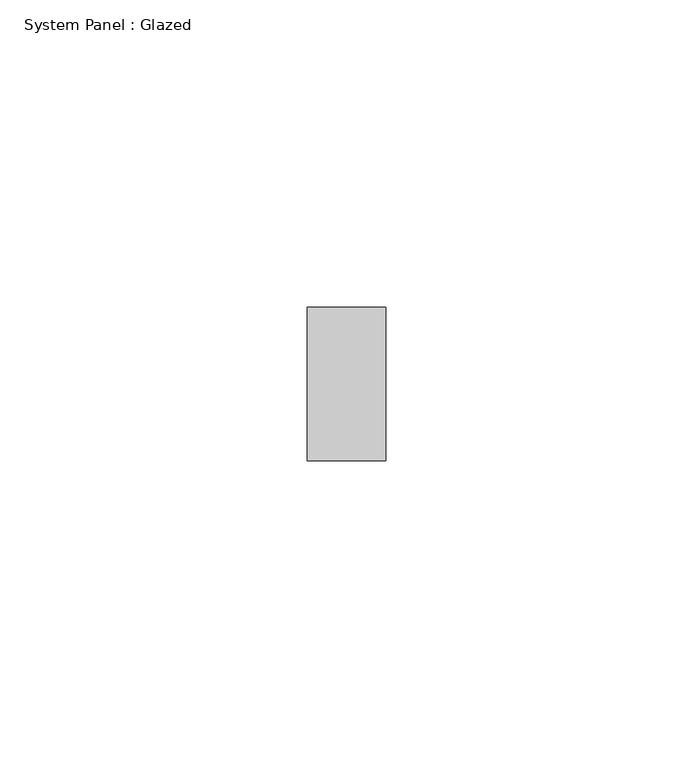
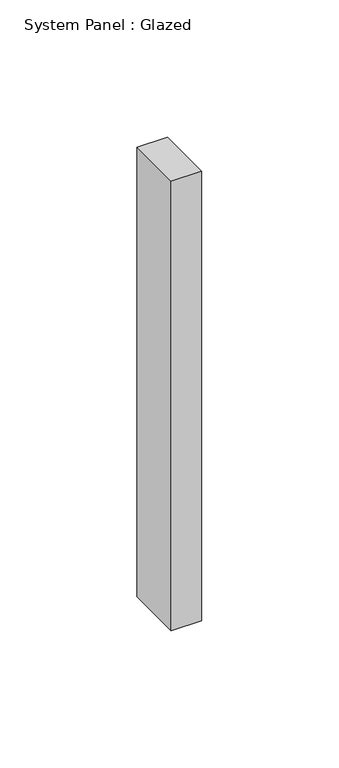
"""IFC4 building model written with IfcOpenShell, lengths in millimetres: plate geometry, System Panel : Glazed."""

from ifc_helpers import new_model, si_unit, origin, origin_with_axes, place, context, project, spatial, polyline, outline, extrude, source, transform, mapped, element, save


def system_panel_glazed_de35cd91(model_context):
    return source(origin(), model_context, "Body", "SweptSolid", [
        extrude(outline(polyline([(6.4022601, 24.5), (-6.4022601, 24.5), (-6.4022601, 49.5), (6.4022601, 49.5), (6.4022601, 24.5)])), origin_with_axes(), (0.0, 0.0, 1.0), 200.0),
    ])


if __name__ == "__main__":
    model = new_model("IFC4")
    model_context = context("Model", 3, world=origin())
    ifc_project = project(units=[si_unit("LENGTHUNIT", "METRE", prefix="MILLI")], contexts=[model_context])
    site = spatial("IfcSite", under=ifc_project)
    building = spatial("IfcBuilding", under=site)
    placement = place(None, origin())
    system_panel_glazed_shape = system_panel_glazed_de35cd91(model_context)
    element("IfcPlate", 1, ObjectType="System Panel : Glazed", at=placement, inside=building, context=model_context, shape_type="MappedRepresentation", body=[
        mapped(system_panel_glazed_shape, transform((0.0, 0.0, 0.0), x_axis=(1.0, 0.0, 0.0), y_axis=(0.0, 1.0, 0.0), z_axis=(0.0, 0.0, 1.0))),
    ])
    save(model, "model.ifc")

# Revit data of these elements
# Element 1 (IfcPlate, "System Panel : Glazed")
#   Materials on its faces: "Glass"
# Materials
#   "Glass": class "Glass", colour RGB 218 227 224, transparency 0.85, Description = "Soda Lime Glass", Cost = 0
